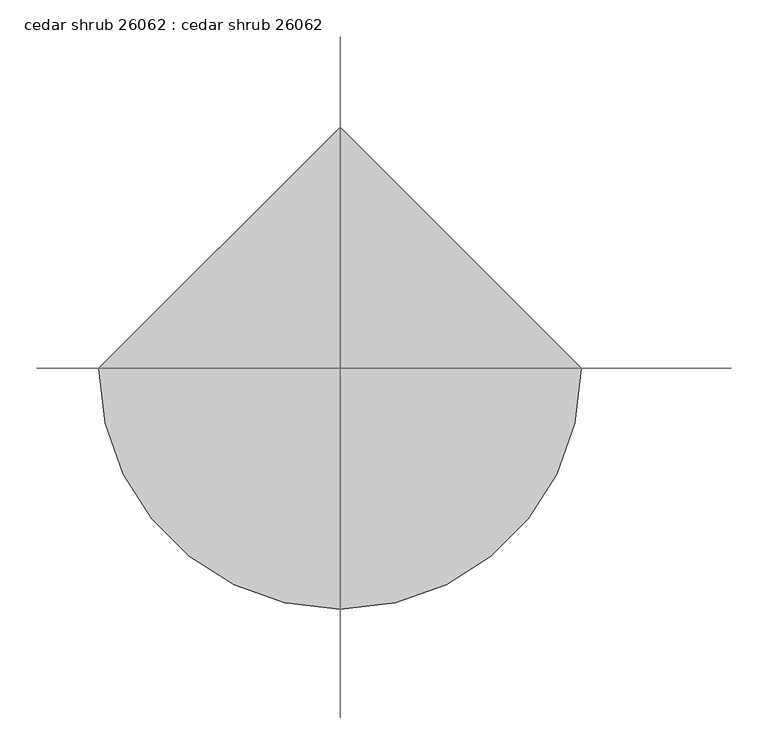
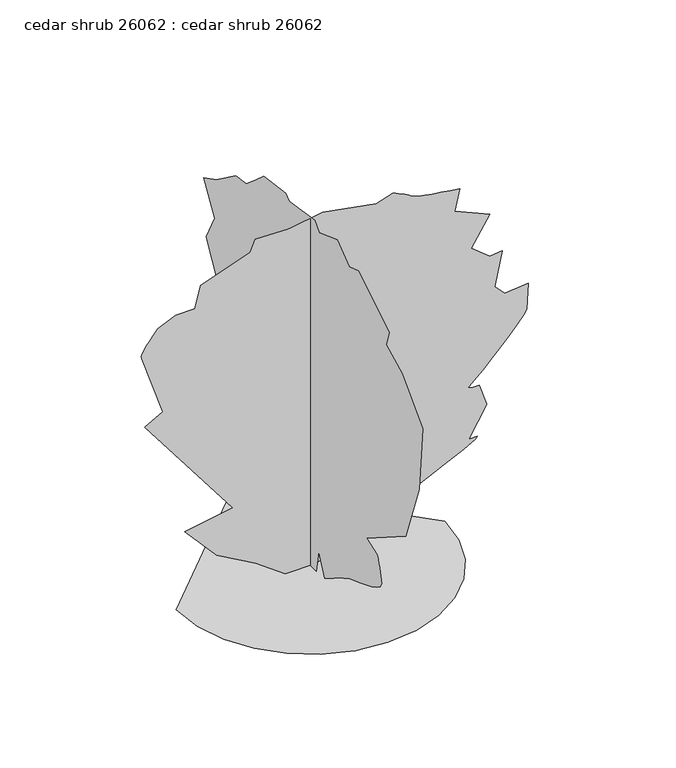
"""IFC4 building model written with IfcOpenShell, lengths in millimetres: proxy geometry, cedar shrub 26062 : cedar shrub 26062."""

from ifc_helpers import new_model, si_unit, origin, place, context, project, spatial, triangles, source, transform, mapped, element, save


def cedar_shrub_26062_cedar_shrub_26062_e27c54a3(model_context):
    return source(origin(), model_context, "Body", "Tessellation", [
        triangles([(-61.9491257, 8.98e-05, 3.1e-06), (-133.3686489, 8.41e-05, 52.0161927), (-229.784339, 7.75e-05, 107.3658847), (-308.3460772, 6.7e-05, 194.8542219), (-190.5039605, 6.45e-05, 216.2798944), (-406.5450977, 3.06e-05, 500.1695792), (-361.9096318, 2.77e-05, 525.1682714), (-413.687576, 9.1e-06, 680.504611), (-414.3708555, 8.5e-06, 686.0316719), (-412.1483531, 7.6e-06, 693.2453304), (-407.5052135, 6.6e-06, 701.8660252), (-400.9240746, 5.4e-06, 711.6120146), (-392.892588, 4.2e-06, 722.1987957), (-383.8933554, 2.8e-06, 733.3493505), (-374.4090142, 1.5e-06, 744.7793941), (-329.7710049, -9e-07, 764.4212185), (-283.347385, -9e-07, 764.4212185), (-269.0649538, -7.7e-06, 821.5560305), (-147.6523519, -1.28e-05, 864.4084293), (-135.1542685, -1.62e-05, 892.975799), (-51.2369207, -1.6e-05, 891.1902248), (30.8950596, -1.77e-05, 905.4726379), (161.2347623, -1.49e-05, 882.2620634), (202.3007514, -1.64e-05, 894.7614458), (209.926594, -1.6e-05, 891.3197227), (217.3964869, -1.56e-05, 887.8932604), (224.5539534, -1.52e-05, 884.4998629), (231.2430618, -1.48e-05, 881.1521021), (237.3073174, -1.44e-05, 877.8678549), (242.5910246, -1.4e-05, 874.6623819), (246.9374708, -1.36e-05, 871.5483278), (253.4703569, -1.33e-05, 868.4368898), (264.8764921, -1.29e-05, 865.2288008), (280.3400286, -1.25e-05, 861.9446262), (299.0547657, -1.21e-05, 858.5968655), (320.205346, -1.17e-05, 855.2034679), (342.9790286, -1.13e-05, 851.779549), (366.5654886, -1.09e-05, 848.337826), (354.0661062, -4.5e-06, 794.774235), (439.7683242, 0.0, 757.2787766), (395.1328583, 8.7e-06, 684.0733612), (439.7683242, 1.3e-05, 648.3660204), (470.1213407, 1.25e-05, 651.9346979), (452.2676702, 2.3e-05, 564.4468695), (477.2638553, 2.59e-05, 539.4507208), (534.3986309, 2.53e-05, 544.8075886), (530.8274099, 3.32e-05, 478.7446515), (523.5757087, 3.45e-05, 467.3451293), (504.7390314, 3.72e-05, 445.2623566), (478.6837177, 4.06e-05, 416.9032228), (449.7886428, 4.42e-05, 386.6696031), (422.4251967, 4.75e-05, 358.9657708), (400.96219, 4.99e-05, 338.196181), (389.7760268, 5.11e-05, 328.7651796), (386.8499336, 5.13e-05, 326.7306381), (386.9235847, 5.15e-05, 325.1634373), (389.4940673, 5.16e-05, 323.9874189), (394.0660629, 5.17e-05, 323.1212654), (400.1341518, 5.18e-05, 322.491362), (407.2029791, 5.19e-05, 322.0189344), (414.7721755, 5.19e-05, 321.622665), (432.6258459, 5.85e-05, 266.2734999), (387.99038, 6.75e-05, 191.2832371), (409.4153077, 6.75e-05, 191.2832371), (404.6121489, 6.81e-05, 185.7135189), (376.0066638, 7e-05, 170.1179047), (327.5713572, 7.28e-05, 146.167468), (263.2661253, 7.65e-05, 115.5335185), (187.0642904, 8.07e-05, 79.8863666), (102.9282468, 8.54e-05, 40.8973356), (14.7802468, 9.02e-05, 3.1e-06), (0.000381, 25.9026863, 6.2e-06), (0.0459126, 34.8300324, 57.3728062), (0.0459011, 134.816453, 119.8644768), (0.045878, 290.1520569, 198.4252067), (0.0458666, 418.7066374, 332.3364006), (0.0458549, 445.4884329, 412.6817508), (0.0458666, 354.4293471, 416.2530081), (0.0458666, 391.9248419, 493.0296444), (0.0458549, 441.9171756, 584.0886938), (0.0458549, 406.2098348, 653.7203447), (0.0458549, 452.6309112, 730.496981), (0.0458549, 400.852967, 757.2787766), (0.0458666, 316.9338161, 817.9848095), (0.0458666, 272.2983865, 825.1272514), (0.0458666, 229.4465145, 860.8371357), (0.045878, 197.3081237, 889.404578), (0.045878, 104.4634274, 901.901417), (0.045878, 90.1794701, 889.404578), (0.0458895, -18.7343943, 907.2582121), (0.0459011, -38.3746062, 885.833357), (0.0459011, -115.1499754, 914.4007267), (0.0459126, -165.1433174, 875.1196215), (0.0459126, -202.6383216, 887.6189312), (0.0459357, -334.7646317, 807.2710739), (0.0459357, -322.2652857, 767.9924395), (0.0459357, -390.1138332, 734.068202), (0.0459474, -477.6016617, 644.7947268), (0.0459588, -463.3167051, 478.7446515), (0.0459474, -404.3962463, 321.622665), (0.0459357, -240.1333076, 216.2798944), (0.0459474, -284.7697909, 200.2108353), (0.0459474, -287.8203315, 191.0282199), (0.0459474, -290.8073766, 181.8458589), (0.0459474, -293.6724997, 172.6634979), (0.0459474, -296.3471184, 163.4808825), (0.0459474, -298.7728243, 154.2985215), (0.0459474, -300.8861037, 145.1161604), (0.0459474, -302.6260048, 135.9335451), (0.0459474, -297.7517384, 125.9028165), (0.0459474, -282.4482212, 114.7161447), (0.0459474, -260.2740114, 103.1860617), (0.0459357, -234.7871223, 92.1246003), (0.0459357, -209.5511809, 82.3433114), (0.0459357, -188.1255083, 74.6549771), (0.0459357, -174.0706613, 69.8711394), (0.0459357, -161.0932739, 63.9628381), (0.0459357, -142.4006376, 53.6509403), (0.0459357, -120.8030006, 40.8714288), (0.0459243, -99.1118918, 27.5610539), (0.0459243, -80.1380772, 15.6561154), (0.0459243, -66.6923272, 7.0931586), (0.0459243, -61.5856531, 3.8085299), (0.0459243, -36.5889844, 59.1581714), (0.0003925, -25.8762707, 0.0), (-329.2655488, 0.0, 9.54e-05), (-320.5609566, -75.445681, 8.64e-05), (-295.7705366, -144.7305826, 7.82e-05), (-256.8780341, -205.8697014, 0.0001171), (-205.8697014, -256.8780341, 0.000111), (-144.7305826, -295.7705366, 0.0001064), (-75.445681, -320.5609566, 0.0001034), (1.15e-05, -329.2655488, 0.0001024), (75.4459354, -320.5609566, 0.0001034), (144.7305826, -295.7705366, 0.0001064), (205.8697014, -256.8780341, 0.000111), (256.8780341, -205.8697014, 0.0001171), (295.7705366, -144.7305826, 7.82e-05), (320.5609566, -75.445681, 8.64e-05), (329.2655488, 2.88e-05, 9.54e-05), (-4.62e-05, 329.2655488, 8.85e-05)], [[63, 64, 65], [63, 65, 66], [3, 4, 5], [42, 43, 44], [45, 46, 47], [5, 6, 7], [39, 40, 41], [37, 38, 39], [2, 3, 5], [45, 47, 48], [45, 48, 49], [36, 37, 39], [60, 61, 62], [19, 20, 21], [59, 60, 62], [59, 62, 63], [58, 59, 63], [57, 58, 63], [56, 57, 63], [45, 49, 50], [17, 18, 19], [35, 36, 39], [45, 50, 51], [44, 45, 51], [44, 51, 52], [41, 42, 44], [23, 24, 25], [34, 35, 39], [44, 52, 53], [41, 44, 53], [41, 53, 54], [41, 54, 55], [1, 2, 5], [71, 1, 5], [70, 71, 5], [69, 70, 5], [68, 69, 5], [68, 5, 7], [67, 68, 7], [66, 67, 7], [63, 66, 7], [56, 63, 7], [55, 56, 7], [41, 55, 7], [39, 41, 7], [34, 39, 7], [33, 34, 7], [32, 33, 7], [31, 32, 7], [30, 31, 7], [29, 30, 7], [28, 29, 7], [27, 28, 7], [26, 27, 7], [25, 26, 7], [23, 25, 7], [22, 23, 7], [21, 22, 7], [19, 21, 7], [17, 19, 7], [17, 7, 8], [16, 17, 8], [15, 16, 8], [14, 15, 8], [13, 14, 8], [12, 13, 8], [11, 12, 8], [10, 11, 8], [9, 10, 8], [76, 77, 78], [122, 123, 124], [81, 82, 83], [121, 122, 124], [124, 125, 72], [124, 72, 73], [75, 76, 78], [120, 121, 124], [94, 95, 96], [93, 94, 96], [91, 92, 93], [119, 120, 124], [89, 90, 91], [79, 80, 81], [101, 102, 103], [81, 83, 84], [81, 84, 85], [97, 98, 99], [87, 88, 89], [96, 97, 99], [74, 75, 78], [96, 99, 100], [96, 100, 101], [93, 96, 101], [91, 93, 101], [89, 91, 101], [87, 89, 101], [86, 87, 101], [85, 86, 101], [81, 85, 101], [79, 81, 101], [78, 79, 101], [74, 78, 101], [73, 74, 101], [124, 73, 101], [119, 124, 101], [118, 119, 101], [117, 118, 101], [116, 117, 101], [115, 116, 101], [114, 115, 101], [113, 114, 101], [112, 113, 101], [112, 101, 103], [112, 103, 104], [112, 104, 105], [111, 112, 105], [111, 105, 106], [111, 106, 107], [110, 111, 107], [110, 107, 108], [109, 110, 108], [140, 141, 126], [139, 140, 126], [139, 126, 127], [138, 139, 127], [138, 127, 128], [138, 128, 129], [137, 138, 129], [136, 137, 129], [136, 129, 130], [136, 130, 131], [136, 131, 132], [136, 132, 133], [136, 133, 134], [136, 134, 135]], closed=False),
    ])


if __name__ == "__main__":
    model = new_model("IFC4")
    model_context = context("Model", 3, world=origin())
    ifc_project = project(units=[si_unit("LENGTHUNIT", "METRE", prefix="MILLI")], contexts=[model_context])
    site = spatial("IfcSite", under=ifc_project)
    building = spatial("IfcBuilding", under=site)
    placement = place(None, origin())
    cedar_shrub_26062_cedar_shrub_26062_shape = cedar_shrub_26062_cedar_shrub_26062_e27c54a3(model_context)
    element("IfcBuildingElementProxy", 1, Name="cedar shrub 26062 : cedar shrub 26062", ObjectType="cedar shrub 26062 : cedar shrub 26062", at=placement, inside=building, context=model_context, shape_type="MappedRepresentation", body=[
        mapped(cedar_shrub_26062_cedar_shrub_26062_shape, transform((0.0, 0.0, 0.0), x_axis=(1.0, 0.0, 0.0), y_axis=(0.0, 1.0, 0.0), z_axis=(0.0, 0.0, 1.0))),
    ])
    save(model, "model.ifc")

# Revit data of these elements
# Type "cedar shrub 26062 : cedar shrub 26062"
#   built-in parameter 1005195 = "RPC-16-FUMD-ULXX-U7X6-J000-ST1L-LVER-AU"
#   Height = 0
